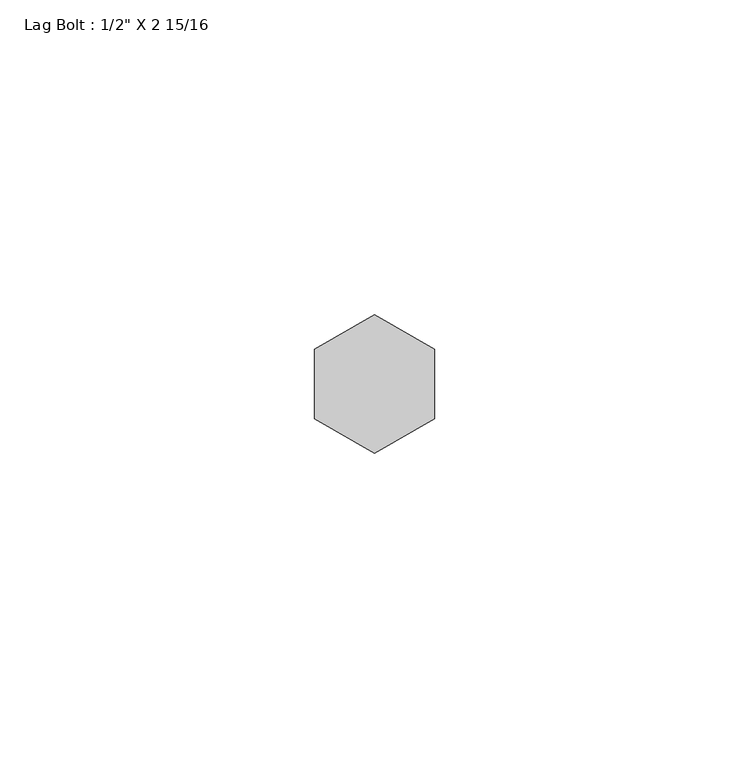
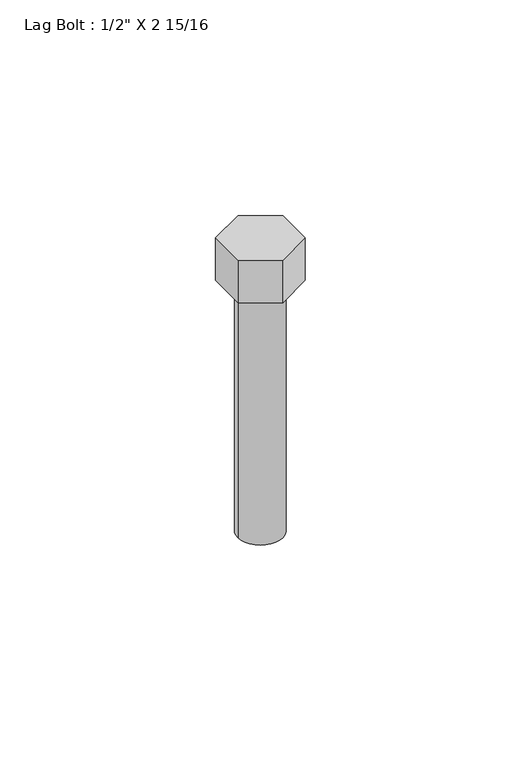
"""IFC4 building model written with IfcOpenShell, lengths in millimetres: proxy geometry."""

import ifcopenshell
import ifcopenshell.guid

model = None  # the IFC model being written
_history = None  # IfcOwnerHistory: only IFC2X3 demands one
_inside = {}  # id of a spatial element -> (the spatial element, [elements in it])
_under = {}  # id of a project, library or spatial element -> (it, [spatial elements below it])
_declared = {}  # id of a project -> (the project, [libraries it declares])
_typed = {}  # id of a type object -> (the type object, [elements of that type])
_made_of = {}  # id of a material, layer set ... -> (it, [elements and type objects made of it])


def new_model(schema):
    """Start an empty IFC model of exactly this schema.

    Asked for "IFC4X3", IfcOpenShell would pick the latest addendum, in which some entities
    have other attributes; the version numbers below select the first issue.
    IFC2X3 requires an IfcOwnerHistory on every rooted entity: one is made here for all.
    """
    global model, _history
    if schema == "IFC4X3":
        model = ifcopenshell.file(schema_version=(4, 3, 0, 0))
    else:
        model = ifcopenshell.file(schema=schema)
    _inside.clear()
    _under.clear()
    _declared.clear()
    _typed.clear()
    _made_of.clear()
    _history = None
    if model.schema == "IFC2X3":
        org = make("IfcOrganization", Name="unknown")
        user = make(
            "IfcPersonAndOrganization",
            ThePerson=make("IfcPerson", FamilyName="unknown"),
            TheOrganization=org,
        )
        app = make(
            "IfcApplication",
            ApplicationDeveloper=org,
            Version="unknown",
            ApplicationFullName="unknown",
            ApplicationIdentifier="unknown",
        )
        _history = make(
            "IfcOwnerHistory",
            OwningUser=user,
            OwningApplication=app,
            ChangeAction="ADDED",
            CreationDate=0,
        )
    return model


def make(cls, **values):
    """One entity of the class cls with the attributes given. An attribute that is None is left unset."""
    return model.create_entity(
        cls, **{name: value for name, value in values.items() if value is not None}
    )


def rooted(cls, **values):
    """An entity with a GlobalId (a new one), such as an element, a storey or a relation."""
    return make(cls, GlobalId=ifcopenshell.guid.new(), OwnerHistory=_history, **values)


def si_unit(unit_type, name, prefix=None):
    """IfcSIUnit, for example si_unit("LENGTHUNIT", "METRE", prefix="MILLI")."""
    return make("IfcSIUnit", UnitType=unit_type, Prefix=prefix, Name=name)


def assignment(units):
    """IfcUnitAssignment: the units of a project."""
    return None if units is None else make("IfcUnitAssignment", Units=units)


def point(xyz):
    """IfcCartesianPoint."""
    return None if xyz is None else make("IfcCartesianPoint", Coordinates=xyz)


def direction(xyz):
    """IfcDirection."""
    return None if xyz is None else make("IfcDirection", DirectionRatios=xyz)


def frame(location, z_axis=None, x_axis=None):
    """IfcAxis2Placement3D, a coordinate frame: its origin and axes. An axis left out is left unset."""
    return make(
        "IfcAxis2Placement3D",
        Location=point(location),
        Axis=direction(z_axis),
        RefDirection=direction(x_axis),
    )


def frame_2d(location, x_axis=None):
    """IfcAxis2Placement2D, a coordinate frame in the plane: its origin and x axis."""
    return make(
        "IfcAxis2Placement2D", Location=point(location), RefDirection=direction(x_axis)
    )


def origin():
    """The frame at (0, 0, 0) with its axes left unset."""
    return frame((0.0, 0.0, 0.0))


def origin_with_axes():
    """The frame at (0, 0, 0) with the z axis (0, 0, 1) and the x axis (1, 0, 0) written out."""
    return frame((0.0, 0.0, 0.0), z_axis=(0.0, 0.0, 1.0), x_axis=(1.0, 0.0, 0.0))


def origin_2d():
    """The frame at (0, 0) in the plane with its x axis left unset."""
    return frame_2d((0.0, 0.0))


def place(relative_to, where):
    """IfcLocalPlacement: puts the frame where relative to a parent placement (None: the world)."""
    return make(
        "IfcLocalPlacement", PlacementRelTo=relative_to, RelativePlacement=where
    )


def context(
    kind, dimensions, precision=None, world=None, true_north=None, identifier=None
):
    """IfcGeometricRepresentationContext, for example the 3D "Model" context."""
    return make(
        "IfcGeometricRepresentationContext",
        ContextIdentifier=identifier,
        ContextType=kind,
        CoordinateSpaceDimension=dimensions,
        Precision=precision,
        WorldCoordinateSystem=world,
        TrueNorth=true_north,
    )


def project(units=None, contexts=None):
    """IfcProject with its units and contexts."""
    return rooted(
        "IfcProject",
        Name="project",
        RepresentationContexts=contexts,
        UnitsInContext=assignment(units),
    )


def spatial(cls, under=None, at=None, **own):
    """A site, building, storey or space (cls), placed at a placement, below another one or the project."""
    s = rooted(cls, ObjectPlacement=at, **own)
    if under is not None:
        _under.setdefault(under.id(), (under, []))[1].append(s)
    return s


def polyline(points):
    """IfcPolyline through the points."""
    return make("IfcPolyline", Points=[point(p) for p in points])


def circle_curve(where, radius):
    """IfcCircle in the frame where."""
    return make("IfcCircle", Position=where, Radius=radius)


def trimmed(basis, trim1, trim2, sense, master):
    """IfcTrimmedCurve: the piece of a basis curve between two trims."""
    return make(
        "IfcTrimmedCurve",
        BasisCurve=basis,
        Trim1=trim1,
        Trim2=trim2,
        SenseAgreement=sense,
        MasterRepresentation=master,
    )


def segment(curve, same_sense, transition):
    """IfcCompositeCurveSegment."""
    return make(
        "IfcCompositeCurveSegment",
        Transition=transition,
        SameSense=same_sense,
        ParentCurve=curve,
    )


def composite_curve(segments, self_intersect=None):
    """IfcCompositeCurve: segments joined end to end."""
    return make("IfcCompositeCurve", Segments=segments, SelfIntersect=self_intersect)


def outline(outer, holes=None, kind="AREA"):
    """IfcArbitraryClosedProfileDef: a profile drawn as a closed curve; with holes, ...WithVoids."""
    if holes is None:
        return make("IfcArbitraryClosedProfileDef", ProfileType=kind, OuterCurve=outer)
    return make(
        "IfcArbitraryProfileDefWithVoids",
        ProfileType=kind,
        OuterCurve=outer,
        InnerCurves=holes,
    )


def extrude(swept, where, along, depth):
    """IfcExtrudedAreaSolid: the profile swept, set in the frame where, extruded along a direction by depth."""
    return make(
        "IfcExtrudedAreaSolid",
        SweptArea=swept,
        Position=where,
        ExtrudedDirection=direction(along),
        Depth=depth,
    )


def shape(context_of_items, identifier, shape_type, items):
    """IfcShapeRepresentation: the items that make up one representation, for example the "Body"."""
    return make(
        "IfcShapeRepresentation",
        ContextOfItems=context_of_items,
        RepresentationIdentifier=identifier,
        RepresentationType=shape_type,
        Items=items,
    )


def source(mapping_origin, context_of_items, identifier, shape_type, items):
    """IfcRepresentationMap: a shape defined once, which mapped items show again and again."""
    return make(
        "IfcRepresentationMap",
        MappingOrigin=mapping_origin,
        MappedRepresentation=shape(context_of_items, identifier, shape_type, items),
    )


def transform(
    local_origin,
    x_axis=None,
    y_axis=None,
    z_axis=None,
    scale=None,
    scale2=None,
    scale3=None,
    uniform=True,
):
    """IfcCartesianTransformationOperator3D, or its non-uniform kind. x_axis, y_axis, z_axis: its Axis1, 2, 3."""
    if uniform:
        return make(
            "IfcCartesianTransformationOperator3D",
            Axis1=direction(x_axis),
            Axis2=direction(y_axis),
            LocalOrigin=point(local_origin),
            Scale=scale,
            Axis3=direction(z_axis),
        )
    return make(
        "IfcCartesianTransformationOperator3DnonUniform",
        Axis1=direction(x_axis),
        Axis2=direction(y_axis),
        LocalOrigin=point(local_origin),
        Scale=scale,
        Axis3=direction(z_axis),
        Scale2=scale2,
        Scale3=scale3,
    )


def mapped(mapping_source, mapping_target):
    """IfcMappedItem: shows the shape of a source again, moved by a transform."""
    return make(
        "IfcMappedItem", MappingSource=mapping_source, MappingTarget=mapping_target
    )


def made_of(thing, what):
    """Note that an element or type object is made of a material, layer set ...; save() writes the relation."""
    if what is not None:
        _made_of.setdefault(what.id(), (what, []))[1].append(thing)
    return thing


def element(
    cls,
    number,
    at=None,
    inside=None,
    cuts=None,
    type_object=None,
    material=None,
    context=None,
    identifier="Body",
    shape_type=None,
    held_by="IfcProductDefinitionShape",
    body=None,
    shapes=None,
    **own,
):
    """One element of the class cls, such as IfcWall. Its Tag is "e" and its number.

    at: its placement. inside: the storey or other place that contains it. cuts: it is an
    opening in that element (IfcRelVoidsElement). A single representation is given by context,
    identifier, shape_type and body (its items); several are given by shapes. held_by: the class
    of the entity that holds the representations. save() writes the other relations.
    """
    e = rooted(cls, Tag="e%d" % number, ObjectPlacement=at, **own)
    if body is not None:
        shapes = [shape(context, identifier, shape_type, body)]
    if shapes is not None:
        e.Representation = make(held_by, Representations=shapes)
    if inside is not None:
        _inside.setdefault(inside.id(), (inside, []))[1].append(e)
    if cuts is not None:
        rooted(
            "IfcRelVoidsElement", RelatingBuildingElement=cuts, RelatedOpeningElement=e
        )
    if type_object is not None:
        _typed.setdefault(type_object.id(), (type_object, []))[1].append(e)
    return made_of(e, material)


def aggregate(whole, parts):
    """IfcRelAggregates: a whole, such as a stair, and the parts it consists of."""
    return rooted("IfcRelAggregates", RelatingObject=whole, RelatedObjects=parts)


def save(model, path):
    """Write the relations noted so far, then the file.

    IfcRelAggregates (storeys below a building ...), IfcRelContainedInSpatialStructure (elements
    in a storey), IfcRelDefinesByType, IfcRelAssociatesMaterial and IfcRelDeclares: one each for
    every whole, place, type object, material and project.
    """
    for whole, parts in _under.values():
        aggregate(whole, parts)
    for where, things in _inside.values():
        rooted(
            "IfcRelContainedInSpatialStructure",
            RelatedElements=things,
            RelatingStructure=where,
        )
    for kind, things in _typed.values():
        rooted("IfcRelDefinesByType", RelatedObjects=things, RelatingType=kind)
    for what, things in _made_of.values():
        rooted("IfcRelAssociatesMaterial", RelatedObjects=things, RelatingMaterial=what)
    for by, libraries in _declared.values():
        rooted("IfcRelDeclares", RelatingContext=by, RelatedDefinitions=libraries)
    model.write(path)


def proxy_0b616378(model_context):
    return source(origin(), model_context, "Body", "SweptSolid", [
        extrude(outline(polyline([(-9.525, -5.4992613), (-9.525, 5.4992613), (0.0, 10.9985226), (9.525, 5.4992613), (9.525, -5.4992613), (0.0, -10.9985226), (-9.525, -5.4992613)])), origin_with_axes(), (0.0, 0.0, 1.0), 12.7),
        extrude(outline(composite_curve([segment(trimmed(circle_curve(origin_2d(), 6.35), [point((-6.35, 0.0))], [point((6.35, 0.0))], False, "CARTESIAN"), True, "CONTINUOUS"), segment(trimmed(circle_curve(origin_2d(), 6.35), [point((6.35, 0.0))], [point((-6.35, 0.0))], False, "CARTESIAN"), True, "CONTINUOUS")], self_intersect=False)), frame((0.0, 0.0, -74.6125), z_axis=(0.0, 0.0, 1.0), x_axis=(1.0, 0.0, 0.0)), (0.0, 0.0, 1.0), 74.6125),
    ])


if __name__ == "__main__":
    model = new_model("IFC4")
    model_context = context("Model", 3, world=origin())
    ifc_project = project(units=[si_unit("LENGTHUNIT", "METRE", prefix="MILLI")], contexts=[model_context])
    site = spatial("IfcSite", under=ifc_project)
    building = spatial("IfcBuilding", under=site)
    placement = place(None, origin())
    proxy_shape = proxy_0b616378(model_context)
    element("IfcBuildingElementProxy", 1, Name="Lag Bolt : 1/2\" X 2 15/16", ObjectType="Lag Bolt : 1/2\" X 2 15/16", at=placement, inside=building, context=model_context, shape_type="MappedRepresentation", body=[
        mapped(proxy_shape, transform((0.0, 0.0, 0.0), x_axis=(1.0, 0.0, 0.0), y_axis=(0.0, 1.0, 0.0), z_axis=(0.0, 0.0, 1.0))),
    ])
    save(model, "model.ifc")

# Revit data of these elements
# Type "Lag Bolt : 1/2\" X 2 15/16"
#   Thickness_of_Substrate [instance default] = 0' - 1"
#   Side = 0' - 0 111/256"
#   Radius = 0' - 0 1/4"
#   Length = 0' - 2 15/16"
#   Head Size = 0' - 0 3/4"
#   Head Radius = 0' - 0 3/8"
#   Head Height = 0' - 0 1/2"
#   Diameter = 0' - 0 1/2"
#   Default Elevation = 4' - 0"
#   Nut_Visibility [instance default] = yes
#   Bolt Material (Size) [instance default] = 1/2" X 5" LAG BOLT (THRU BOLT IF PLATE ON OPP. SIDE OF STRUCT MEMBER)
# Element 1 (IfcBuildingElementProxy, "Lag Bolt : 1/2\" X 2 15/16")
#   Nut_Visibility = no
#   Bolt Material (Size) = THRU-BOLT OR LAG BOLT
#   Materials on its faces: "THRU-BOLT OR LAG BOLT"
# Materials
#   "1/2\" X 5\" LAG BOLT (THRU BOLT IF PLATE ON OPP. SIDE OF STRUCT MEMBER)": class "Generic", colour RGB 120 120 120, transparency 0, Cost = 0
#   "THRU-BOLT OR LAG BOLT": class "Generic", colour RGB 120 120 120, transparency 0, Cost = 0
